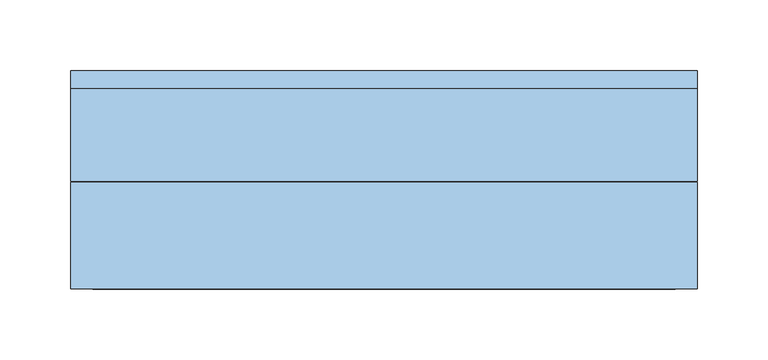
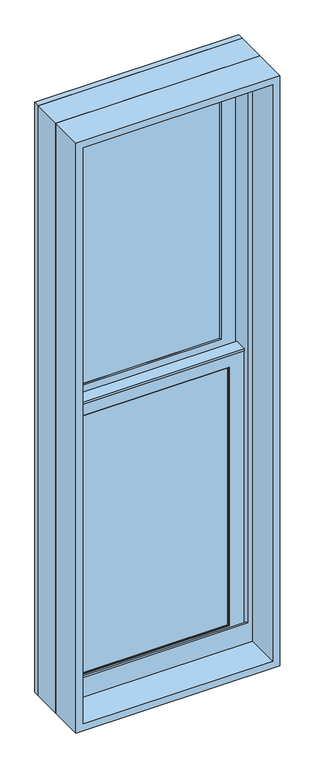
"""IFC4 building model written with IfcOpenShell, lengths in millimetres: window geometry, Window-Double_Hung-Marvin-Essential : ESDH1646."""

from ifc_helpers import new_model, si_unit, frame, origin, place, context, project, spatial, polyline, outline, extrude, faceted_brep, source, transform, mapped, element, save


def window_9e9364bf(model_context):
    return source(origin(), model_context, "Body", "SolidModel", [
        extrude(outline(polyline([(64.5583333, 20.6375), (64.5583333, 15.875), (45.5083333, 15.875), (45.5083333, 20.6375), (64.5583333, 20.6375)])), frame((0.0, 0.0, 1136.65), z_axis=(0.0, 0.0, 1.0), x_axis=(1.0, 0.0, 0.0)), (0.0, 0.0, 1.0), 603.25),
        extrude(outline(polyline([(-45.5083333, 20.6375), (-45.5083333, 15.875), (-64.5583333, 15.875), (-64.5583333, 20.6375), (-45.5083333, 20.6375)])), frame((0.0, 0.0, 1136.65), z_axis=(0.0, 0.0, 1.0), x_axis=(1.0, 0.0, 0.0)), (0.0, 0.0, 1.0), 603.25),
        extrude(outline(polyline([(165.1, 20.6375), (165.1, 15.875), (-165.1, 15.875), (-165.1, 20.6375), (165.1, 20.6375)])), frame((0.0, 0.0, 1428.75), z_axis=(0.0, 0.0, 1.0), x_axis=(1.0, 0.0, 0.0)), (0.0, 0.0, 1.0), 19.05),
        extrude(outline(polyline([(-64.5583333, 46.83125), (-64.5583333, 51.59375), (-45.5083333, 51.59375), (-45.5083333, 46.83125), (-64.5583333, 46.83125)])), frame((0.0, 0.0, 1778.0), z_axis=(0.0, 0.0, 1.0), x_axis=(1.0, 0.0, 0.0)), (0.0, 0.0, 1.0), 603.25),
        extrude(outline(polyline([(45.5083333, 46.83125), (45.5083333, 51.59375), (64.5583333, 51.59375), (64.5583333, 46.83125), (45.5083333, 46.83125)])), frame((0.0, 0.0, 1778.0), z_axis=(0.0, 0.0, 1.0), x_axis=(1.0, 0.0, 0.0)), (0.0, 0.0, 1.0), 603.25),
        extrude(outline(polyline([(-165.1, 46.83125), (-165.1, 51.59375), (165.1, 51.59375), (165.1, 46.83125), (-165.1, 46.83125)])), frame((0.0, 0.0, 2070.1), z_axis=(0.0, 0.0, 1.0), x_axis=(1.0, 0.0, 0.0)), (0.0, 0.0, 1.0), 19.05),
        extrude(outline(polyline([(64.5583333, 20.6375), (45.5083333, 20.6375), (45.5083333, 25.4), (64.5583333, 25.4), (64.5583333, 20.6375)])), frame((0.0, 0.0, 1136.65), z_axis=(0.0, 0.0, 1.0), x_axis=(1.0, 0.0, 0.0)), (0.0, 0.0, 1.0), 603.25),
        extrude(outline(polyline([(-45.5083333, 20.6375), (-64.5583333, 20.6375), (-64.5583333, 25.4), (-45.5083333, 25.4), (-45.5083333, 20.6375)])), frame((0.0, 0.0, 1136.65), z_axis=(0.0, 0.0, 1.0), x_axis=(1.0, 0.0, 0.0)), (0.0, 0.0, 1.0), 603.25),
        extrude(outline(polyline([(165.1, 20.6375), (-165.1, 20.6375), (-165.1, 25.4), (165.1, 25.4), (165.1, 20.6375)])), frame((0.0, 0.0, 1428.75), z_axis=(0.0, 0.0, 1.0), x_axis=(1.0, 0.0, 0.0)), (0.0, 0.0, 1.0), 19.05),
        extrude(outline(polyline([(-64.5583333, 56.35625), (-45.5083333, 56.35625), (-45.5083333, 51.59375), (-64.5583333, 51.59375), (-64.5583333, 56.35625)])), frame((0.0, 0.0, 1778.0), z_axis=(0.0, 0.0, 1.0), x_axis=(1.0, 0.0, 0.0)), (0.0, 0.0, 1.0), 603.25),
        extrude(outline(polyline([(45.5083333, 56.35625), (64.5583333, 56.35625), (64.5583333, 51.59375), (45.5083333, 51.59375), (45.5083333, 56.35625)])), frame((0.0, 0.0, 1778.0), z_axis=(0.0, 0.0, 1.0), x_axis=(1.0, 0.0, 0.0)), (0.0, 0.0, 1.0), 603.25),
        extrude(outline(polyline([(-165.1, 56.35625), (165.1, 56.35625), (165.1, 51.59375), (-165.1, 51.59375), (-165.1, 56.35625)])), frame((0.0, 0.0, 2070.1), z_axis=(0.0, 0.0, 1.0), x_axis=(1.0, 0.0, 0.0)), (0.0, 0.0, 1.0), 19.05),
        faceted_brep([(-192.0875, 5.6780605, 1769.9351748), (-192.0875, 5.6780605, 1765.3), (192.0875, 5.6780605, 1765.3), (192.0875, 5.6780605, 1769.9351748), (-192.0875, 34.8118605, 1769.9351748), (192.0875, 34.8118605, 1769.9351748), (192.0875, 34.8118605, 1765.3), (-192.0875, 34.8118605, 1765.3), (-192.0875, 30.1625, 1765.3), (-192.0875, 30.1625, 1109.6625), (-192.0875, 8.9241104, 1109.6625), (-192.0875, 8.9241104, 1765.3), (192.0875, 8.9241104, 1765.3), (192.0875, 30.1625, 1765.3), (192.0875, 8.9241104, 1109.6625), (192.0875, 30.1625, 1109.6625), (-176.2034752, 11.90625, 1751.0034752), (-176.2034752, 30.1625, 1751.0034752), (176.2034752, 30.1625, 1751.0034752), (176.2034752, 11.90625, 1751.0034752), (-159.54375, 10.4662439, 1734.34375), (-159.54375, 11.90625, 1734.34375), (159.54375, 11.90625, 1734.34375), (159.54375, 10.4662439, 1734.34375), (161.0858834, 8.9241104, 1735.8858834), (-161.0858834, 8.9241104, 1735.8858834), (176.2034752, 30.1625, 1125.5465248), (176.2034752, 11.90625, 1125.5465248), (159.54375, 11.90625, 1142.20625), (159.54375, 10.4662439, 1142.20625), (161.0858834, 8.9241104, 1140.6641166), (-176.2034752, 30.1625, 1125.5465248), (-176.2034752, 11.90625, 1125.5465248), (-159.54375, 11.90625, 1142.20625), (-159.54375, 10.4662439, 1142.20625), (-161.0858834, 8.9241104, 1140.6641166)], [[[0, 1, 2, 3]], [[4, 5, 6, 7]], [[1, 0, 4, 7, 8, 9, 10, 11]], [[2, 1, 11, 12]], [[7, 6, 13, 8]], [[3, 2, 12, 14, 15, 13, 6, 5]], [[0, 3, 5, 4]], [[16, 17, 18, 19]], [[20, 21, 22, 23]], [[20, 23, 24, 25]], [[19, 18, 26, 27]], [[23, 22, 28, 29]], [[24, 23, 29, 30]], [[27, 26, 31, 32]], [[29, 28, 33, 34]], [[30, 29, 34, 35]], [[15, 14, 10, 9]], [[15, 9, 8, 13], [18, 17, 31, 26]], [[17, 16, 32, 31]], [[16, 19, 27, 32], [22, 21, 33, 28]], [[21, 20, 34, 33]], [[20, 25, 35, 34]], [[10, 14, 12, 11], [25, 24, 30, 35]]]),
        extrude(outline(polyline([(38.5955581, 1751.0125), (33.5778968, 1751.0125), (33.5778968, 1752.6), (39.9405976, 1752.6), (39.9405976, 1751.0125), (61.515625, 1751.0125), (47.6307501, 1747.6975159), (38.5955581, 1747.6975159), (38.5955581, 1751.0125)])), frame((-192.0875, 0.0, 0.0), z_axis=(1.0, 0.0, 0.0), x_axis=(0.0, 1.0, 0.0)), (0.0, 0.0, 1.0), 384.175),
        faceted_brep([(222.25, 0.0, 1079.5), (222.25, 0.0, 2438.4), (-222.25, 0.0, 2438.4), (-222.25, 0.0, 1079.5), (196.05625, 0.0, 1140.61875), (-196.05625, 0.0, 1140.61875), (-196.05625, 0.0, 2412.20625), (196.05625, 0.0, 2412.20625), (196.05625, 3.96875, 1079.5), (-196.05625, 3.96875, 1079.5), (-196.05625, 3.96875, 1140.61875), (196.05625, 3.96875, 1140.61875), (-222.25, 65.6828125, 1079.5), (-196.05625, 65.6828125, 1079.5), (196.05625, 65.6828125, 1079.5), (222.25, 65.6828125, 1079.5), (-222.25, 65.6828125, 2438.4), (222.25, 65.6828125, 2438.4), (196.05625, 65.6828125, 2412.20625), (-196.05625, 65.6828125, 2412.20625)], [[[0, 1, 2, 3], [4, 5, 6, 7]], [[8, 9, 10, 11]], [[5, 4, 11, 10]], [[0, 3, 12, 13, 9, 8, 14, 15]], [[13, 12, 16, 17, 15, 14, 18, 19]], [[13, 19, 6, 5, 10, 9]], [[7, 6, 19, 18]], [[18, 14, 8, 11, 4, 7]], [[1, 0, 15, 17]], [[2, 1, 17, 16]], [[3, 2, 16, 12]]]),
        faceted_brep([(196.05625, 30.1625, 1758.95), (194.46875, 30.1625, 1758.95), (194.46875, 30.1625, 1103.8544613), (196.05625, 30.1625, 1103.8544613), (-194.46875, 30.1625, 1758.95), (-196.05625, 30.1625, 1758.95), (-196.05625, 30.1625, 1103.8544613), (-194.46875, 30.1625, 1103.8544613), (194.46875, 63.5, 1758.95), (196.05625, 63.5, 1758.95), (196.05625, 63.5, 1097.3743077), (194.46875, 63.5, 1097.3743077), (-196.05625, 63.5, 1758.95), (-194.46875, 63.5, 1758.95), (-194.46875, 63.5, 1097.3743077), (-196.05625, 63.5, 1097.3743077), (207.3108932, 3.96875, 1108.9460105), (207.3108932, 3.96875, 1079.5), (207.3108932, 65.6828125, 1079.5), (207.3108932, 65.6828125, 1096.950012), (-207.3108932, 3.96875, 1079.5), (-207.3108932, 3.96875, 1108.9460105), (-207.3108932, 65.6828125, 1096.950012), (-207.3108932, 65.6828125, 1079.5), (207.3108932, 78.58125, 1094.4428097), (-207.3108932, 78.58125, 1094.4428097), (-205.2971252, 68.2348864, 1096.4539391), (-187.33135, 68.2348864, 1096.4539391), (-187.33135, 65.6828125, 1096.950012), (187.33135, 65.6828125, 1096.950012), (187.33135, 68.2348864, 1096.4539391), (205.2971252, 68.2348864, 1096.4539391), (-222.25, 65.6828125, 1079.5), (-222.25, 78.5948249, 1079.5), (222.25, 78.5948249, 1079.5), (222.25, 65.6828125, 1079.5), (-222.25, 78.58125, 2438.4), (222.25, 78.58125, 2438.4), (207.3108932, 78.58125, 2423.4608932), (-207.3108932, 78.58125, 2423.4608932), (-222.25, 65.6828125, 2438.4), (-205.2971252, 68.2348864, 2421.4471252), (205.2971252, 68.2348864, 2421.4471252), (187.33135, 68.2348864, 2403.48135), (-187.33135, 68.2348864, 2403.48135), (-187.33135, 65.6828125, 2403.48135), (187.33135, 65.6828125, 2403.48135), (222.25, 65.6828125, 2438.4)], [[[0, 1, 2, 3]], [[4, 5, 6, 7]], [[8, 9, 10, 11]], [[12, 13, 14, 15]], [[1, 8, 11, 2]], [[9, 0, 3, 10]], [[1, 0, 9, 8]], [[5, 4, 13, 12]], [[5, 12, 15, 6]], [[13, 4, 7, 14]], [[16, 17, 18, 19]], [[20, 21, 22, 23]], [[24, 25, 26, 27, 28, 22, 21, 16, 19, 29, 30, 31], [3, 2, 11, 10], [7, 6, 15, 14]], [[17, 16, 21, 20]], [[17, 20, 23, 32, 33, 34, 35, 18]], [[34, 33, 36, 37], [25, 24, 38, 39]], [[33, 32, 40, 36]], [[39, 41, 26, 25]], [[41, 42, 31, 30, 43, 44, 27, 26]], [[44, 45, 28, 27]], [[40, 32, 23, 22, 28, 45, 46, 29, 19, 18, 35, 47]], [[36, 40, 47, 37]], [[39, 38, 42, 41]], [[44, 43, 46, 45]], [[34, 37, 47, 35]], [[42, 38, 24, 31]], [[46, 43, 30, 29]]]),
        extrude(outline(polyline([(172.24375, 11.90625), (-172.24375, 11.90625), (-172.24375, 15.08125), (172.24375, 15.08125), (172.24375, 11.90625)])), frame((0.0, 0.0, 1129.50625), z_axis=(0.0, 0.0, 1.0), x_axis=(1.0, 0.0, 0.0)), (0.0, 0.0, 1.0), 617.5375),
        extrude(outline(polyline([(172.24375, 42.8625), (-172.24375, 42.8625), (-172.24375, 46.0375), (172.24375, 46.0375), (172.24375, 42.8625)])), frame((0.0, 0.0, 1770.85625), z_axis=(0.0, 0.0, 1.0), x_axis=(1.0, 0.0, 0.0)), (0.0, 0.0, 1.0), 617.5375),
        faceted_brep([(-159.54375, 31.194477, 1734.34375), (-161.0858834, 32.7366104, 1735.8858834), (161.0858834, 32.7366104, 1735.8858834), (159.54375, 31.194477, 1734.34375), (-159.54375, 30.1625, 1734.34375), (159.54375, 30.1625, 1734.34375), (-192.0875, 32.7366104, 1766.8875), (-192.0875, 30.1625, 1766.8875), (192.0875, 30.1625, 1766.8875), (192.0875, 32.7366104, 1766.8875), (161.0858834, 32.7366104, 1140.6641166), (159.54375, 31.194477, 1142.20625), (159.54375, 30.1625, 1142.20625), (192.0875, 30.1625, 1109.6625), (192.0875, 32.7366104, 1109.6625), (-161.0858834, 32.7366104, 1140.6641166), (-159.54375, 31.194477, 1142.20625), (-159.54375, 30.1625, 1142.20625), (-192.0875, 30.1625, 1109.6625), (-192.0875, 32.7366104, 1109.6625)], [[[0, 1, 2, 3]], [[4, 0, 3, 5]], [[6, 7, 8, 9]], [[3, 2, 10, 11]], [[5, 3, 11, 12]], [[9, 8, 13, 14]], [[11, 10, 15, 16]], [[12, 11, 16, 17]], [[14, 13, 18, 19]], [[9, 14, 19, 6], [1, 15, 10, 2]], [[16, 15, 1, 0]], [[17, 16, 0, 4]], [[7, 18, 13, 8], [5, 12, 17, 4]], [[19, 18, 7, 6]]]),
        faceted_brep([(-176.2034752, 42.8625, 2392.3534752), (-176.2034752, 61.11875, 2392.3534752), (176.2034752, 61.11875, 2392.3534752), (176.2034752, 42.8625, 2392.3534752), (-159.54375, 41.4224939, 2375.69375), (-159.54375, 42.8625, 2375.69375), (159.54375, 42.8625, 2375.69375), (159.54375, 41.4224939, 2375.69375), (-161.0858834, 39.8803604, 2377.2358834), (161.0858834, 39.8803604, 2377.2358834), (-192.0875, 61.11875, 2408.2375), (-192.0875, 39.8803604, 2408.2375), (192.0875, 39.8803604, 2408.2375), (192.0875, 61.11875, 2408.2375), (176.2034752, 61.11875, 1766.8965248), (176.2034752, 42.8625, 1766.8965248), (159.54375, 42.8625, 1783.55625), (159.54375, 41.4224939, 1783.55625), (161.0858834, 39.8803604, 1782.0141166), (192.0875, 39.8803604, 1751.0125), (192.0875, 61.11875, 1751.0125), (-176.2034752, 61.11875, 1766.8965248), (-176.2034752, 42.8625, 1766.8965248), (-159.54375, 42.8625, 1783.55625), (-159.54375, 41.4224939, 1783.55625), (-161.0858834, 39.8803604, 1782.0141166), (-192.0875, 39.8803604, 1751.0125), (-192.0875, 61.11875, 1751.0125)], [[[0, 1, 2, 3]], [[4, 5, 6, 7]], [[8, 4, 7, 9]], [[10, 11, 12, 13]], [[3, 2, 14, 15]], [[7, 6, 16, 17]], [[9, 7, 17, 18]], [[13, 12, 19, 20]], [[15, 14, 21, 22]], [[17, 16, 23, 24]], [[18, 17, 24, 25]], [[20, 19, 26, 27]], [[13, 20, 27, 10], [1, 21, 14, 2]], [[22, 21, 1, 0]], [[3, 15, 22, 0], [5, 23, 16, 6]], [[24, 23, 5, 4]], [[25, 24, 4, 8]], [[11, 26, 19, 12], [9, 18, 25, 8]], [[27, 26, 11, 10]]]),
        faceted_brep([(-192.0875, 61.11875, 1751.0125), (-192.0875, 63.6928604, 1751.0125), (192.0875, 63.6928604, 1751.0125), (192.0875, 61.11875, 1751.0125), (-159.54375, 62.150727, 1783.55625), (-159.54375, 61.11875, 1783.55625), (159.54375, 61.11875, 1783.55625), (159.54375, 62.150727, 1783.55625), (-161.0858834, 63.6928604, 1782.0141166), (161.0858834, 63.6928604, 1782.0141166), (192.0875, 63.6928604, 2408.2375), (192.0875, 61.11875, 2408.2375), (159.54375, 61.11875, 2375.69375), (159.54375, 62.150727, 2375.69375), (161.0858834, 63.6928604, 2377.2358834), (-192.0875, 63.6928604, 2408.2375), (-192.0875, 61.11875, 2408.2375), (-159.54375, 61.11875, 2375.69375), (-159.54375, 62.150727, 2375.69375), (-161.0858834, 63.6928604, 2377.2358834)], [[[0, 1, 2, 3]], [[4, 5, 6, 7]], [[8, 4, 7, 9]], [[3, 2, 10, 11]], [[7, 6, 12, 13]], [[9, 7, 13, 14]], [[11, 10, 15, 16]], [[13, 12, 17, 18]], [[14, 13, 18, 19]], [[16, 15, 1, 0]], [[3, 11, 16, 0], [5, 17, 12, 6]], [[18, 17, 5, 4]], [[19, 18, 4, 8]], [[1, 15, 10, 2], [9, 14, 19, 8]]]),
        extrude(outline(polyline([(172.24375, 26.19375), (-172.24375, 26.19375), (-172.24375, 30.1625), (172.24375, 30.1625), (172.24375, 26.19375)])), frame((0.0, 0.0, 1129.50625), z_axis=(0.0, 0.0, 1.0), x_axis=(1.0, 0.0, 0.0)), (0.0, 0.0, 1.0), 617.5375),
        extrude(outline(polyline([(172.24375, 57.15), (-172.24375, 57.15), (-172.24375, 61.11875), (172.24375, 61.11875), (172.24375, 57.15)])), frame((0.0, 0.0, 1770.85625), z_axis=(0.0, 0.0, 1.0), x_axis=(1.0, 0.0, 0.0)), (0.0, 0.0, 1.0), 617.5375),
        extrude(outline(polyline([(2438.4, 222.25), (2438.4, -222.25), (1079.5, -222.25), (1079.5, 222.25), (2438.4, 222.25)]), holes=[polyline([(2422.525, 206.375), (1095.375, 206.375), (1095.375, -206.375), (2422.525, -206.375), (2422.525, 206.375)])]), frame((0.0, -76.2, 0.0), z_axis=(0.0, 1.0, 0.0), x_axis=(0.0, 0.0, 1.0)), (0.0, 0.0, 1.0), 75.40625),
    ])


if __name__ == "__main__":
    model = new_model("IFC4")
    model_context = context("Model", 3, world=origin())
    ifc_project = project(units=[si_unit("LENGTHUNIT", "METRE", prefix="MILLI")], contexts=[model_context])
    site = spatial("IfcSite", under=ifc_project)
    building = spatial("IfcBuilding", under=site)
    placement = place(None, origin())
    window_shape = window_9e9364bf(model_context)
    element("IfcWindow", 1, ObjectType="Window-Double_Hung-Marvin-Essential : ESDH1646", at=placement, inside=building, context=model_context, shape_type="MappedRepresentation", body=[
        mapped(window_shape, transform((0.0, 0.0, 0.0), x_axis=(1.0, 0.0, 0.0), y_axis=(0.0, 1.0, 0.0), z_axis=(0.0, 0.0, 1.0))),
    ])
    save(model, "model.ifc")

# Revit data of these elements
# Type "Window-Double_Hung-Marvin-Essential : ESDH1646"
#   Type Mark = "54"
#   Window Type = "Essential Double Hung"
#   Product data url = "https://bimobject.com/marvin-windows-and-doors/product/marvin-dhwau"
#   Product Guid = "c4a96547-874c-4385-91dc-a058adc19d98"
#   Frame = "All Ultrex"
#   Egress Window = "No"
#   URL = "www.marvin.com"
#   Model = "ESDH1646"
#   Manufacturer = "Marvin Windows and Doors"
#   Label Egress = ""
#   Glass Type = "IG Low E II with Argon"
#   Design Pressure = "DP50"
#   Description = "1854 DBHG"
#   Analytic Construction = "<None>"
#   Prairie Corner Width = 0' - 4"
#   Prairie Corner Height = 0' - 4"
#   Egress Width = 1' - 2 9/16"
#   Egress Height = 1' - 10 27/128"
#   Rough Width = 1' - 6"
#   Rough Height = 4' - 6"
#   Nominal Width = 1' - 6"
#   Nominal Height = 4' - 6"
#   Inset to Installation Flange [instance default] = 0' - 1"
#   Height = 4' - 5 1/2"
#   Egress Area = 2.24616 SF
#   Default Head Height = 8' - 0"
#   Width = 1' - 5 1/2"
#   Daylight Area = 4.06755 SF
#   DLO Width = 1' - 0 9/16"
#   DLO Height = 1' - 11 5/16"
#   Muntins Top Sash = yes
#   Lites Wide Top Sash = 3
#   Lites Wide Bottom Sash = 3
#   Lites High Top Sash = 2
#   Lites High Bottom Sash = 2
#   Lite Cut Prairie 9 = no
#   Lite Cut HV Grid = yes
#   Muntins Bottom Sash = yes
#   Label Visibility = no
#   Jamb Extension Visibility = yes
#   Edition number = 1
#   Interior Material = Ultrex-Marvin-Stonewhite
#   Glazing Material = Glass-Marvin-IG Low E II with Argon
#   Cladding Material = Ultrex-Marvin-Pebblegray
#   Wall Closure = (empty or 0)
#   Assembly Code = ""
# Element 1 (IfcWindow, "Window-Double_Hung-Marvin-Essential : ESDH1646")
#   Materials on its faces: "Ultrex-Marvin-Pebblegray", "Ultrex-Marvin-Stonewhite", "Glass-Marvin-IG Low E II with Argon"
# Materials
#   "Ultrex-Marvin-Stonewhite": class "Paint", colour RGB 250 251 245, transparency 0
#   "Glass-Marvin-IG Low E II with Argon": class "Glass", colour RGB 0 128 192, transparency 0.85
#   "Ultrex-Marvin-Pebblegray": class "Paint", colour RGB 189 185 173, transparency 0
